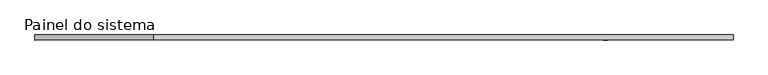
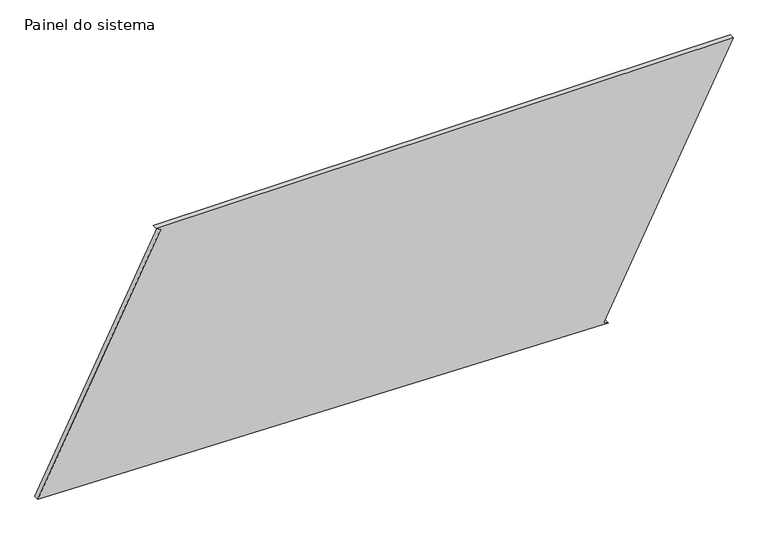
"""IFC4 building model written with IfcOpenShell, lengths in millimetres: plate geometry, Painel do sistema : Envidraçado."""

from ifc_helpers import new_model, si_unit, frame, origin, place, context, project, spatial, polyline, outline, extrude, source, transform, mapped, element, save


def painel_do_sistema_581223ec(model_context):
    return source(origin(), model_context, "Body", "SweptSolid", [
        extrude(outline(polyline([(0.0, 1101.7464331), (11.291819, 1079.4418411), (1277.5710966, 1720.5024959), (1277.5710966, -1134.9957546), (1266.2792777, -1112.6911626), (65.6769784, -1720.5024959), (0.0, 1101.7464331)])), frame((0.0, 24.5, 0.0), z_axis=(0.0, 1.0, 0.0), x_axis=(0.0, 0.0, 1.0)), (0.0, 0.0, 1.0), 25.0),
    ])


if __name__ == "__main__":
    model = new_model("IFC4")
    model_context = context("Model", 3, world=origin())
    ifc_project = project(units=[si_unit("LENGTHUNIT", "METRE", prefix="MILLI")], contexts=[model_context])
    site = spatial("IfcSite", under=ifc_project)
    building = spatial("IfcBuilding", under=site)
    placement = place(None, origin())
    painel_do_sistema_shape = painel_do_sistema_581223ec(model_context)
    element("IfcPlate", 1, ObjectType="Painel do sistema : Envidraçado", at=placement, inside=building, context=model_context, shape_type="MappedRepresentation", body=[
        mapped(painel_do_sistema_shape, transform((0.0, 0.0, 0.0), x_axis=(1.0, 0.0, 0.0), y_axis=(0.0, 1.0, 0.0), z_axis=(0.0, 0.0, 1.0))),
    ])
    save(model, "model.ifc")

# Revit data of these elements
# Type "Painel do sistema : Envidraçado"
#   Construction Type Id = "GSP4R"
#   Analytic Construction = "Vidraça única Pilkington 1/8 pol"
#   Visual Light Transmittance = 0.9
#   Solar Heat Gain Coefficient = 0.86
#   Heat Transfer Coefficient (U) = 6.7069 W/(m²·K)
# Element 1 (IfcPlate, "Painel do sistema : Envidraçado")
#   Materials on its faces: "Vidro"
# Materials
#   "Vidro": class "Vidro", colour RGB 0 128 192, transparency 0.9, Description = "Vidro de sílica", Cost = 0
